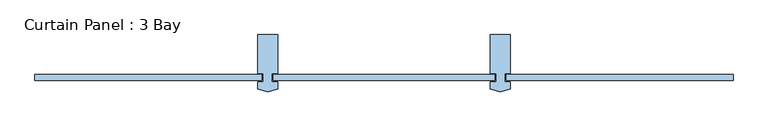
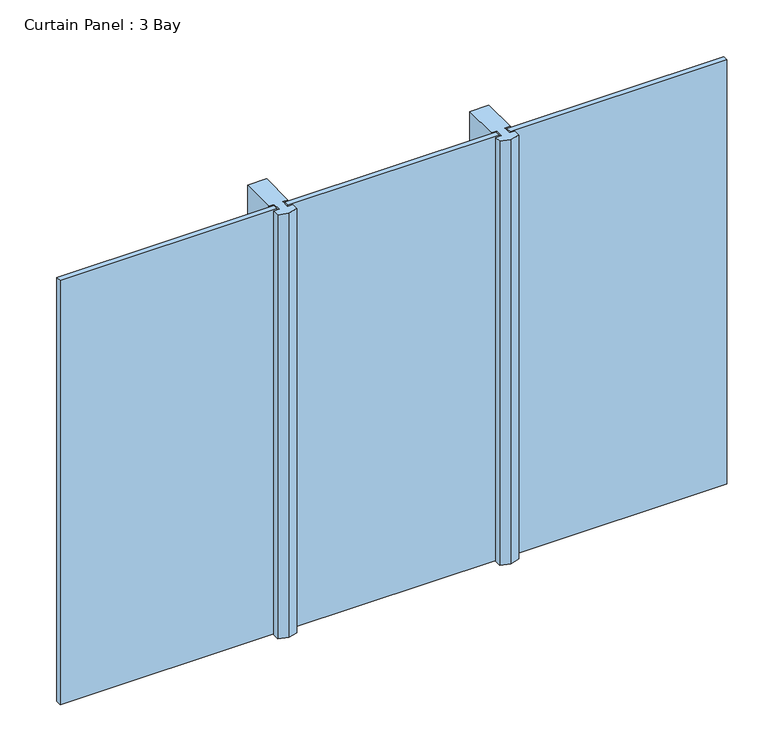
"""IFC4 building model written with IfcOpenShell, lengths in millimetres: window geometry, Curtain Panel : 3 Bay."""

from ifc_helpers import new_model, si_unit, origin, origin_with_axes, place, context, project, spatial, polyline, outline, extrude, source, transform, mapped, element, save


def curtain_panel_3_bay_d95054c0(model_context):
    return source(origin(), model_context, "Body", "SweptSolid", [
        extrude(outline(polyline([(-472.0166667, -12.7), (-497.4166667, -12.7), (-497.4166667, -50.8), (-472.0166667, -50.8), (-472.0166667, -82.55), (-516.4666667, -95.25), (-560.9166667, -82.55), (-560.9166667, -50.8), (-535.5166667, -50.8), (-535.5166667, -12.7), (-560.9166667, -12.7), (-560.9166667, 158.75), (-472.0166667, 158.75), (-472.0166667, -12.7)])), origin_with_axes(), (0.0, 0.0, 1.0), 2085.3785982),
        extrude(outline(polyline([(472.0166667, -12.7), (472.0166667, 158.75), (560.9166667, 158.75), (560.9166667, -12.7), (535.5166667, -12.7), (535.5166667, -50.8), (560.9166667, -50.8), (560.9166667, -82.55), (516.4666667, -95.25), (472.0166667, -82.55), (472.0166667, -50.8), (497.4166667, -50.8), (497.4166667, -12.7), (472.0166667, -12.7)])), origin_with_axes(), (0.0, 0.0, 1.0), 2085.3785982),
        extrude(outline(polyline([(-491.0666667, -44.45), (-491.0666667, -19.05), (491.0666667, -19.05), (491.0666667, -44.45), (-491.0666667, -44.45)])), origin_with_axes(), (0.0, 0.0, 1.0), 2085.3785982),
        extrude(outline(polyline([(-1549.4, -44.45), (-1549.4, -19.05), (-541.8666667, -19.05), (-541.8666667, -44.45), (-1549.4, -44.45)])), origin_with_axes(), (0.0, 0.0, 1.0), 2085.3785982),
        extrude(outline(polyline([(541.8666667, -44.45), (541.8666667, -19.05), (1549.4, -19.05), (1549.4, -44.45), (541.8666667, -44.45)])), origin_with_axes(), (0.0, 0.0, 1.0), 2085.3785982),
    ])


if __name__ == "__main__":
    model = new_model("IFC4")
    model_context = context("Model", 3, world=origin())
    ifc_project = project(units=[si_unit("LENGTHUNIT", "METRE", prefix="MILLI")], contexts=[model_context])
    site = spatial("IfcSite", under=ifc_project)
    building = spatial("IfcBuilding", under=site)
    placement = place(None, origin())
    curtain_panel_3_bay_shape = curtain_panel_3_bay_d95054c0(model_context)
    element("IfcWindow", 1, ObjectType="Curtain Panel : 3 Bay", at=placement, inside=building, context=model_context, shape_type="MappedRepresentation", body=[
        mapped(curtain_panel_3_bay_shape, transform((0.0, 0.0, 0.0), x_axis=(1.0, 0.0, 0.0), y_axis=(0.0, 1.0, 0.0), z_axis=(0.0, 0.0, 1.0))),
    ])
    save(model, "model.ifc")

# Revit data of these elements
# Type "Curtain Panel : 3 Bay"
#   Type Mark = "24"
#   Description = "The Aubin Academy Master Series"
#   Offset = 0' - 1 1/4"
# Element 1 (IfcWindow, "Curtain Panel : 3 Bay")
#   Materials on its faces: "Metal - Aluminum", "Glass"
# Materials
#   "Metal - Aluminum": class "Metal", colour RGB 247 247 247, transparency 0
#   "Glass": class "Glass", colour RGB 0 128 192, transparency 0.75, Description = "Soda Lime Glass", Cost = 0
